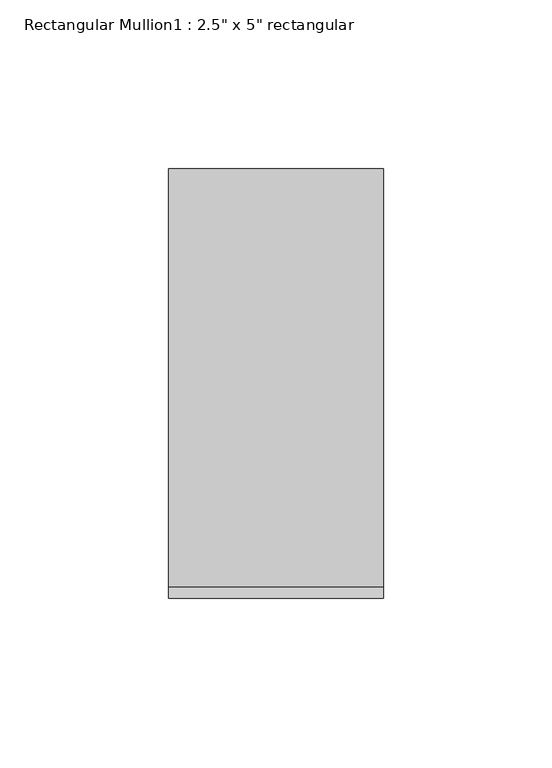
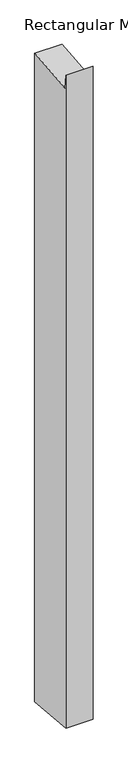
"""IFC4 building model written with IfcOpenShell, lengths in millimetres: member geometry."""

from ifc_helpers import new_model, si_unit, frame, origin, place, context, project, spatial, polyline, outline, extrude, source, transform, mapped, element, save


def member_c2dac231(model_context):
    return source(origin(), model_context, "Body", "SweptSolid", [
        extrude(outline(polyline([(-63.5, 28.7582861), (-60.2336356, -5.8295375), (63.5, 5.8554747), (63.5, -1598.9426588), (-63.5, -1586.9491815), (-63.5, 28.7582861)])), frame((-63.5, 0.0, 0.0), z_axis=(1.0, 0.0, 0.0), x_axis=(0.0, 1.0, 0.0)), (0.0, 0.0, 1.0), 63.5),
    ])


if __name__ == "__main__":
    model = new_model("IFC4")
    model_context = context("Model", 3, world=origin())
    ifc_project = project(units=[si_unit("LENGTHUNIT", "METRE", prefix="MILLI")], contexts=[model_context])
    site = spatial("IfcSite", under=ifc_project)
    building = spatial("IfcBuilding", under=site)
    placement = place(None, origin())
    member_shape = member_c2dac231(model_context)
    element("IfcMember", 1, ObjectType="Rectangular Mullion1 : 2.5\" x 5\" rectangular", at=placement, inside=building, context=model_context, shape_type="MappedRepresentation", body=[
        mapped(member_shape, transform((0.0, 0.0, 0.0), x_axis=(1.0, 0.0, 0.0), y_axis=(0.0, 1.0, 0.0), z_axis=(0.0, 0.0, 1.0))),
    ])
    save(model, "model.ifc")

# Revit data of these elements
# Type "Rectangular Mullion1 : 2.5\" x 5\" rectangular"
#   built-in parameter 1007304 = 0.416667 (stored number, unit not read)
#   built-in parameter 1007301 = 0.104167 (stored number, unit not read)
#   built-in parameter 1007300 = 0.104167 (stored number, unit not read)
# Element 1 (IfcMember, "Rectangular Mullion1 : 2.5\" x 5\" rectangular")
#   Materials on its faces: "support-frame"
# Materials
#   "support-frame": class "Unassigned", colour RGB 233 233 233, transparency 0, Cost = 0
